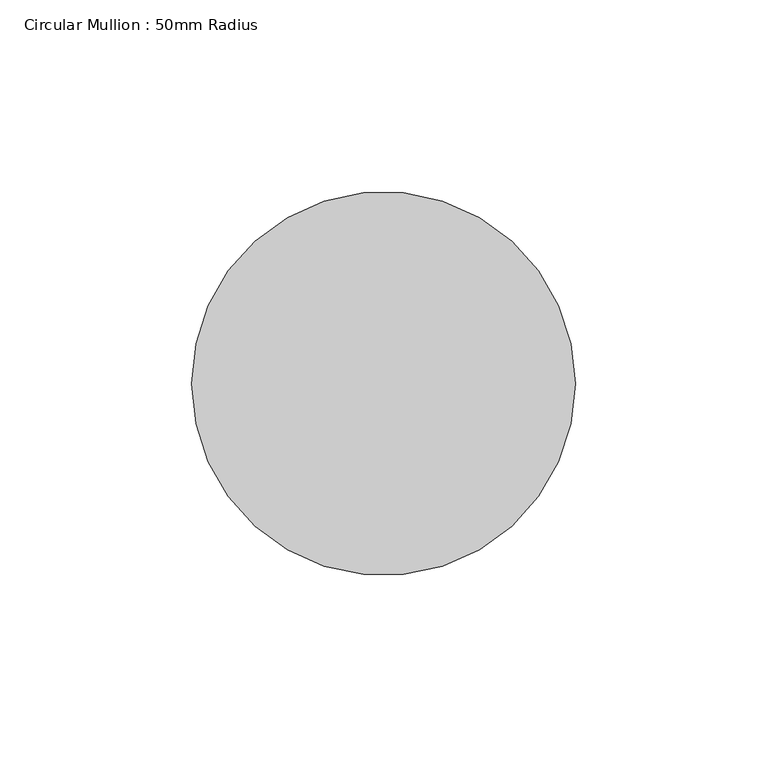
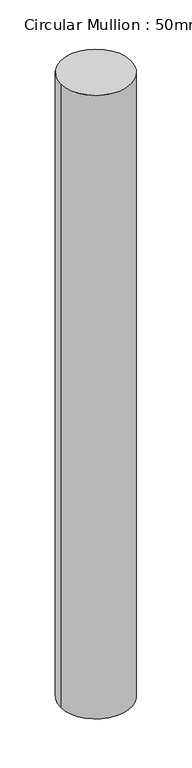
"""IFC4 building model written with IfcOpenShell, lengths in millimetres: member geometry, Circular Mullion : 50mm Radius."""

from ifc_helpers import new_model, si_unit, point, frame, origin, origin_2d, place, context, project, spatial, circle_curve, trimmed, segment, composite_curve, outline, extrude, source, transform, mapped, element, save


def circular_mullion_50mm_radius_46c61cfd(model_context):
    return source(origin(), model_context, "Body", "SweptSolid", [
        extrude(outline(composite_curve([segment(trimmed(circle_curve(origin_2d(), 50.0), [point((50.0, 0.0))], [point((-50.0, 0.0))], False, "CARTESIAN"), True, "CONTINUOUS"), segment(trimmed(circle_curve(origin_2d(), 50.0), [point((-50.0, 0.0))], [point((50.0, 0.0))], False, "CARTESIAN"), True, "CONTINUOUS")], self_intersect=False)), frame((0.0, 0.0, -939.2152922), z_axis=(0.0, 0.0, 1.0), x_axis=(1.0, 0.0, 0.0)), (0.0, 0.0, 1.0), 939.2152922),
    ])


if __name__ == "__main__":
    model = new_model("IFC4")
    model_context = context("Model", 3, world=origin())
    ifc_project = project(units=[si_unit("LENGTHUNIT", "METRE", prefix="MILLI")], contexts=[model_context])
    site = spatial("IfcSite", under=ifc_project)
    building = spatial("IfcBuilding", under=site)
    placement = place(None, origin())
    circular_mullion_50mm_radius_shape = circular_mullion_50mm_radius_46c61cfd(model_context)
    element("IfcMember", 1, ObjectType="Circular Mullion : 50mm Radius", at=placement, inside=building, context=model_context, shape_type="MappedRepresentation", body=[
        mapped(circular_mullion_50mm_radius_shape, transform((0.0, 0.0, 0.0), x_axis=(1.0, 0.0, 0.0), y_axis=(0.0, 1.0, 0.0), z_axis=(0.0, 0.0, 1.0))),
    ])
    save(model, "model.ifc")

# Revit data of these elements
# Type "Circular Mullion : 50mm Radius"
#   built-in parameter 1007350 = 0.164042 (stored number, unit not read)
# Element 1 (IfcMember, "Circular Mullion : 50mm Radius")
#   Materials on its faces: "Aluminium"
# Materials
#   "Aluminium": class "Metal", colour RGB 247 247 247, transparency 0, Description = "Aluminium 6061", Cost = 0
